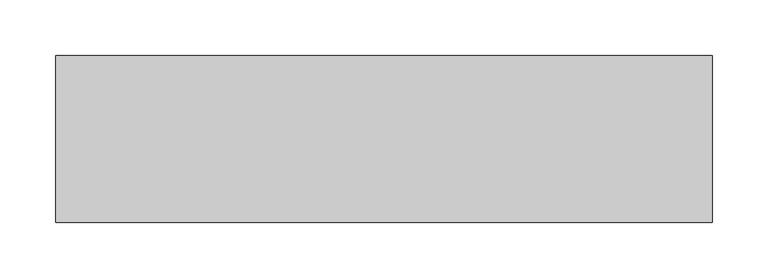
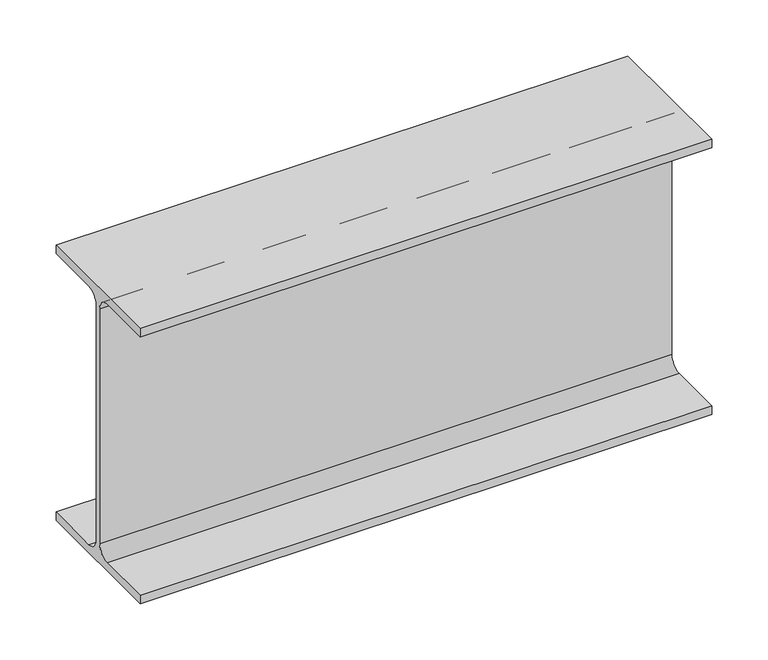
"""IFC4 building model written with IfcOpenShell, lengths in millimetres: beam geometry, 0912_Steel Framing_H-KSD3502 : H_SB_ASB_H-300x150x6.5x9."""

import ifcopenshell
import ifcopenshell.guid

model = None  # the IFC model being written
_history = None  # IfcOwnerHistory: only IFC2X3 demands one
_inside = {}  # id of a spatial element -> (the spatial element, [elements in it])
_under = {}  # id of a project, library or spatial element -> (it, [spatial elements below it])
_declared = {}  # id of a project -> (the project, [libraries it declares])
_typed = {}  # id of a type object -> (the type object, [elements of that type])
_made_of = {}  # id of a material, layer set ... -> (it, [elements and type objects made of it])


def new_model(schema):
    """Start an empty IFC model of exactly this schema.

    Asked for "IFC4X3", IfcOpenShell would pick the latest addendum, in which some entities
    have other attributes; the version numbers below select the first issue.
    IFC2X3 requires an IfcOwnerHistory on every rooted entity: one is made here for all.
    """
    global model, _history
    if schema == "IFC4X3":
        model = ifcopenshell.file(schema_version=(4, 3, 0, 0))
    else:
        model = ifcopenshell.file(schema=schema)
    _inside.clear()
    _under.clear()
    _declared.clear()
    _typed.clear()
    _made_of.clear()
    _history = None
    if model.schema == "IFC2X3":
        org = make("IfcOrganization", Name="unknown")
        user = make(
            "IfcPersonAndOrganization",
            ThePerson=make("IfcPerson", FamilyName="unknown"),
            TheOrganization=org,
        )
        app = make(
            "IfcApplication",
            ApplicationDeveloper=org,
            Version="unknown",
            ApplicationFullName="unknown",
            ApplicationIdentifier="unknown",
        )
        _history = make(
            "IfcOwnerHistory",
            OwningUser=user,
            OwningApplication=app,
            ChangeAction="ADDED",
            CreationDate=0,
        )
    return model


def make(cls, **values):
    """One entity of the class cls with the attributes given. An attribute that is None is left unset."""
    return model.create_entity(
        cls, **{name: value for name, value in values.items() if value is not None}
    )


def rooted(cls, **values):
    """An entity with a GlobalId (a new one), such as an element, a storey or a relation."""
    return make(cls, GlobalId=ifcopenshell.guid.new(), OwnerHistory=_history, **values)


def si_unit(unit_type, name, prefix=None):
    """IfcSIUnit, for example si_unit("LENGTHUNIT", "METRE", prefix="MILLI")."""
    return make("IfcSIUnit", UnitType=unit_type, Prefix=prefix, Name=name)


def assignment(units):
    """IfcUnitAssignment: the units of a project."""
    return None if units is None else make("IfcUnitAssignment", Units=units)


def point(xyz):
    """IfcCartesianPoint."""
    return None if xyz is None else make("IfcCartesianPoint", Coordinates=xyz)


def direction(xyz):
    """IfcDirection."""
    return None if xyz is None else make("IfcDirection", DirectionRatios=xyz)


def frame(location, z_axis=None, x_axis=None):
    """IfcAxis2Placement3D, a coordinate frame: its origin and axes. An axis left out is left unset."""
    return make(
        "IfcAxis2Placement3D",
        Location=point(location),
        Axis=direction(z_axis),
        RefDirection=direction(x_axis),
    )


def frame_2d(location, x_axis=None):
    """IfcAxis2Placement2D, a coordinate frame in the plane: its origin and x axis."""
    return make(
        "IfcAxis2Placement2D", Location=point(location), RefDirection=direction(x_axis)
    )


def origin():
    """The frame at (0, 0, 0) with its axes left unset."""
    return frame((0.0, 0.0, 0.0))


def place(relative_to, where):
    """IfcLocalPlacement: puts the frame where relative to a parent placement (None: the world)."""
    return make(
        "IfcLocalPlacement", PlacementRelTo=relative_to, RelativePlacement=where
    )


def context(
    kind, dimensions, precision=None, world=None, true_north=None, identifier=None
):
    """IfcGeometricRepresentationContext, for example the 3D "Model" context."""
    return make(
        "IfcGeometricRepresentationContext",
        ContextIdentifier=identifier,
        ContextType=kind,
        CoordinateSpaceDimension=dimensions,
        Precision=precision,
        WorldCoordinateSystem=world,
        TrueNorth=true_north,
    )


def project(units=None, contexts=None):
    """IfcProject with its units and contexts."""
    return rooted(
        "IfcProject",
        Name="project",
        RepresentationContexts=contexts,
        UnitsInContext=assignment(units),
    )


def spatial(cls, under=None, at=None, **own):
    """A site, building, storey or space (cls), placed at a placement, below another one or the project."""
    s = rooted(cls, ObjectPlacement=at, **own)
    if under is not None:
        _under.setdefault(under.id(), (under, []))[1].append(s)
    return s


def polyline(points):
    """IfcPolyline through the points."""
    return make("IfcPolyline", Points=[point(p) for p in points])


def circle_curve(where, radius):
    """IfcCircle in the frame where."""
    return make("IfcCircle", Position=where, Radius=radius)


def trimmed(basis, trim1, trim2, sense, master):
    """IfcTrimmedCurve: the piece of a basis curve between two trims."""
    return make(
        "IfcTrimmedCurve",
        BasisCurve=basis,
        Trim1=trim1,
        Trim2=trim2,
        SenseAgreement=sense,
        MasterRepresentation=master,
    )


def segment(curve, same_sense, transition):
    """IfcCompositeCurveSegment."""
    return make(
        "IfcCompositeCurveSegment",
        Transition=transition,
        SameSense=same_sense,
        ParentCurve=curve,
    )


def composite_curve(segments, self_intersect=None):
    """IfcCompositeCurve: segments joined end to end."""
    return make("IfcCompositeCurve", Segments=segments, SelfIntersect=self_intersect)


def outline(outer, holes=None, kind="AREA"):
    """IfcArbitraryClosedProfileDef: a profile drawn as a closed curve; with holes, ...WithVoids."""
    if holes is None:
        return make("IfcArbitraryClosedProfileDef", ProfileType=kind, OuterCurve=outer)
    return make(
        "IfcArbitraryProfileDefWithVoids",
        ProfileType=kind,
        OuterCurve=outer,
        InnerCurves=holes,
    )


def extrude(swept, where, along, depth):
    """IfcExtrudedAreaSolid: the profile swept, set in the frame where, extruded along a direction by depth."""
    return make(
        "IfcExtrudedAreaSolid",
        SweptArea=swept,
        Position=where,
        ExtrudedDirection=direction(along),
        Depth=depth,
    )


def shape(context_of_items, identifier, shape_type, items):
    """IfcShapeRepresentation: the items that make up one representation, for example the "Body"."""
    return make(
        "IfcShapeRepresentation",
        ContextOfItems=context_of_items,
        RepresentationIdentifier=identifier,
        RepresentationType=shape_type,
        Items=items,
    )


def source(mapping_origin, context_of_items, identifier, shape_type, items):
    """IfcRepresentationMap: a shape defined once, which mapped items show again and again."""
    return make(
        "IfcRepresentationMap",
        MappingOrigin=mapping_origin,
        MappedRepresentation=shape(context_of_items, identifier, shape_type, items),
    )


def transform(
    local_origin,
    x_axis=None,
    y_axis=None,
    z_axis=None,
    scale=None,
    scale2=None,
    scale3=None,
    uniform=True,
):
    """IfcCartesianTransformationOperator3D, or its non-uniform kind. x_axis, y_axis, z_axis: its Axis1, 2, 3."""
    if uniform:
        return make(
            "IfcCartesianTransformationOperator3D",
            Axis1=direction(x_axis),
            Axis2=direction(y_axis),
            LocalOrigin=point(local_origin),
            Scale=scale,
            Axis3=direction(z_axis),
        )
    return make(
        "IfcCartesianTransformationOperator3DnonUniform",
        Axis1=direction(x_axis),
        Axis2=direction(y_axis),
        LocalOrigin=point(local_origin),
        Scale=scale,
        Axis3=direction(z_axis),
        Scale2=scale2,
        Scale3=scale3,
    )


def mapped(mapping_source, mapping_target):
    """IfcMappedItem: shows the shape of a source again, moved by a transform."""
    return make(
        "IfcMappedItem", MappingSource=mapping_source, MappingTarget=mapping_target
    )


def made_of(thing, what):
    """Note that an element or type object is made of a material, layer set ...; save() writes the relation."""
    if what is not None:
        _made_of.setdefault(what.id(), (what, []))[1].append(thing)
    return thing


def element(
    cls,
    number,
    at=None,
    inside=None,
    cuts=None,
    type_object=None,
    material=None,
    context=None,
    identifier="Body",
    shape_type=None,
    held_by="IfcProductDefinitionShape",
    body=None,
    shapes=None,
    **own,
):
    """One element of the class cls, such as IfcWall. Its Tag is "e" and its number.

    at: its placement. inside: the storey or other place that contains it. cuts: it is an
    opening in that element (IfcRelVoidsElement). A single representation is given by context,
    identifier, shape_type and body (its items); several are given by shapes. held_by: the class
    of the entity that holds the representations. save() writes the other relations.
    """
    e = rooted(cls, Tag="e%d" % number, ObjectPlacement=at, **own)
    if body is not None:
        shapes = [shape(context, identifier, shape_type, body)]
    if shapes is not None:
        e.Representation = make(held_by, Representations=shapes)
    if inside is not None:
        _inside.setdefault(inside.id(), (inside, []))[1].append(e)
    if cuts is not None:
        rooted(
            "IfcRelVoidsElement", RelatingBuildingElement=cuts, RelatedOpeningElement=e
        )
    if type_object is not None:
        _typed.setdefault(type_object.id(), (type_object, []))[1].append(e)
    return made_of(e, material)


def aggregate(whole, parts):
    """IfcRelAggregates: a whole, such as a stair, and the parts it consists of."""
    return rooted("IfcRelAggregates", RelatingObject=whole, RelatedObjects=parts)


def save(model, path):
    """Write the relations noted so far, then the file.

    IfcRelAggregates (storeys below a building ...), IfcRelContainedInSpatialStructure (elements
    in a storey), IfcRelDefinesByType, IfcRelAssociatesMaterial and IfcRelDeclares: one each for
    every whole, place, type object, material and project.
    """
    for whole, parts in _under.values():
        aggregate(whole, parts)
    for where, things in _inside.values():
        rooted(
            "IfcRelContainedInSpatialStructure",
            RelatedElements=things,
            RelatingStructure=where,
        )
    for kind, things in _typed.values():
        rooted("IfcRelDefinesByType", RelatedObjects=things, RelatingType=kind)
    for what, things in _made_of.values():
        rooted("IfcRelAssociatesMaterial", RelatedObjects=things, RelatingMaterial=what)
    for by, libraries in _declared.values():
        rooted("IfcRelDeclares", RelatingContext=by, RelatedDefinitions=libraries)
    model.write(path)


def beam_8e0ea4b8(model_context):
    return source(origin(), model_context, "Body", "SweptSolid", [
        extrude(outline(composite_curve([segment(polyline([(-75.0, -141.0), (-16.25, -141.0)]), True, "CONTINUOUS"), segment(trimmed(circle_curve(frame_2d((-16.25, -128.0)), 13.0), [point((-16.25, -141.0))], [point((-3.25, -128.0))], True, "CARTESIAN"), True, "CONTINUOUS"), segment(polyline([(-3.25, -128.0), (-3.25, 128.0)]), True, "CONTINUOUS"), segment(trimmed(circle_curve(frame_2d((-16.25, 128.0)), 13.0), [point((-3.25, 128.0))], [point((-16.25, 141.0))], True, "CARTESIAN"), True, "CONTINUOUS"), segment(polyline([(-16.25, 141.0), (-75.0, 141.0), (-75.0, 150.0), (75.0, 150.0), (75.0, 141.0), (16.25, 141.0)]), True, "CONTINUOUS"), segment(trimmed(circle_curve(frame_2d((16.25, 128.0)), 13.0), [point((16.25, 141.0))], [point((3.25, 128.0))], True, "CARTESIAN"), True, "CONTINUOUS"), segment(polyline([(3.25, 128.0), (3.25, -128.0)]), True, "CONTINUOUS"), segment(trimmed(circle_curve(frame_2d((16.25, -128.0)), 13.0), [point((3.25, -128.0))], [point((16.25, -141.0))], True, "CARTESIAN"), True, "CONTINUOUS"), segment(polyline([(16.25, -141.0), (75.0, -141.0), (75.0, -150.0), (-75.0, -150.0), (-75.0, -141.0)]), True, "CONTINUOUS")], self_intersect=False)), frame((-282.3, 0.0, 0.0), z_axis=(1.0, 0.0, 0.0), x_axis=(0.0, 1.0, 0.0)), (0.0, 0.0, 1.0), 589.6),
    ])


if __name__ == "__main__":
    model = new_model("IFC4")
    model_context = context("Model", 3, world=origin())
    ifc_project = project(units=[si_unit("LENGTHUNIT", "METRE", prefix="MILLI")], contexts=[model_context])
    site = spatial("IfcSite", under=ifc_project)
    building = spatial("IfcBuilding", under=site)
    placement = place(None, origin())
    beam_shape = beam_8e0ea4b8(model_context)
    element("IfcBeam", 1, ObjectType="0912_Steel Framing_H-KSD3502 : H_SB_ASB_H-300x150x6.5x9", at=placement, inside=building, context=model_context, shape_type="MappedRepresentation", body=[
        mapped(beam_shape, transform((0.0, 0.0, 0.0), x_axis=(1.0, 0.0, 0.0), y_axis=(0.0, 1.0, 0.0), z_axis=(0.0, 0.0, 1.0))),
    ])
    save(model, "model.ifc")

# Revit data of these elements
# Type "0912_Steel Framing_H-KSD3502 : H_SB_ASB_H-300x150x6.5x9"
#   H_WM Code_1 = "S01AA002-00001 | Main Steel Structure Fabrication Work | Shelter/Building | Medium Steel - Standard (90KG/M>Weight≥30KG/M) | Material: (   )"
#   H_WM Code_2 = "S03AA028-00001 | Main Steel Structure Erection Work | Shelter/Building | Medium Steel (90KG/M>Weight≥30KG/M) | Material: (   )"
#   H_WM Code_3 = "S01AA010-00001 | Main Steel Structure Fabrication Work | Shelter/Building | Steel Painting/Coating | for Non-Fireproofed Steel Surface, Surface Preparation, Primer, Second & Final Coat | Material: (   )"
#   H_Q'ty Cal Type Tag = "SB-Q2"
#   Width = 15.0 cm
#   Web Thickness = 0.65 cm
#   Web Fillet = 1.3 cm
#   Warping Constant = 107000.0 cm⁶
#   W = 0
#   Torsional Moment of Inertia = 9.9539 cm⁴
#   Section Area = 46.78 cm²
#   Plastic Modulus weak axis = 105.0 cm³
#   Plastic Modulus strong axis = 542.0 cm³
#   Perimeter = 1.17 m²/m
#   Nominal Weight = 36.70 kgf/m
#   Moment of Inertia weak axis = 508.00 cm⁴
#   Moment of Inertia strong axis = 7210.00 cm⁴
#   Height = 30.0 cm
#   Flange Thickness = 0.9 cm
#   Elastic Modulus weak axis = 67.7 cm³
#   Elastic Modulus strong axis = 481.0 cm³
#   Centroid Vertical = 15.0 cm
#   Centroid Horizontal = 7.5 cm
#   Ix = 72100000
#   Length [instance default] = 1.5240 m
#   Zx = 542000
#   b = 0.1500 m
#   h = 0.3000 m
#   r = 0.0130 m
#   s = 0.0065 m
#   t = 0.0090 m
#   A = 0.004678 m²
#   Structural Material [instance default] = Steel, 45-345
#   Assembly Code = ""
# Element 1 (IfcBeam, "0912_Steel Framing_H-KSD3502 : H_SB_ASB_H-300x150x6.5x9")
#   Structural Material = none
# Materials
#   "Steel, 45-345": class "Metal", colour RGB 189 187 185, transparency 0, Description = "Steel 345 MPa", Cost = 0
